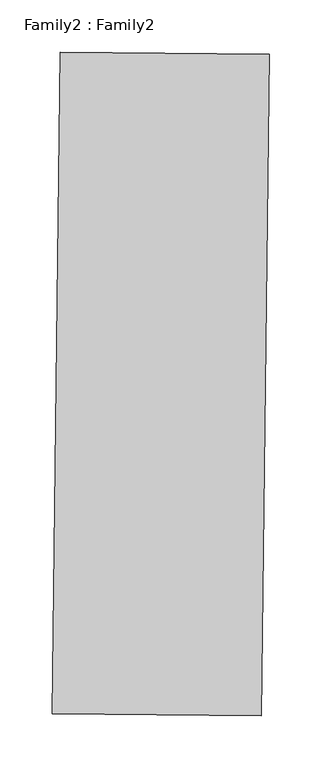
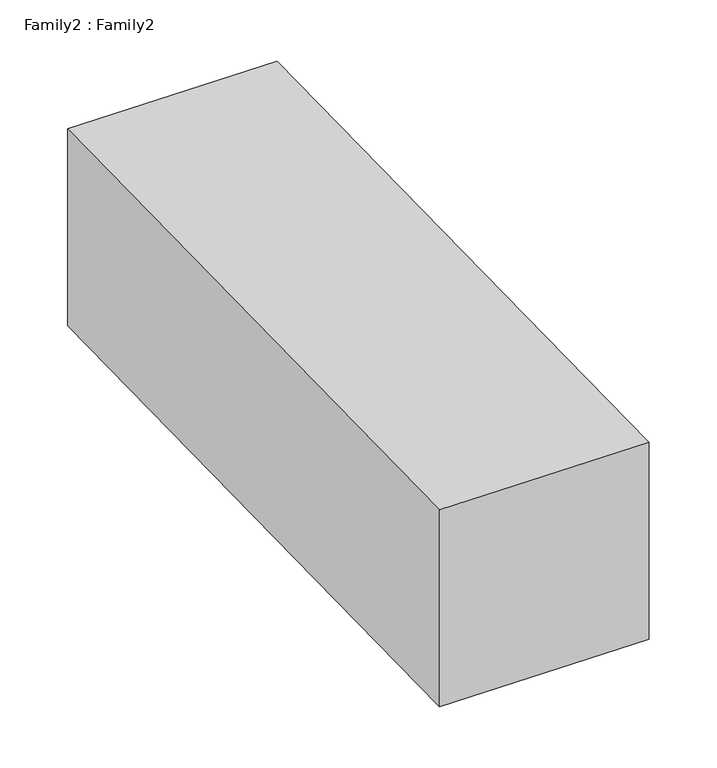
"""IFC4 building model written with IfcOpenShell, lengths in millimetres: proxy geometry, Family2 : Family2."""

import ifcopenshell
import ifcopenshell.guid

model = None  # the IFC model being written
_history = None  # IfcOwnerHistory: only IFC2X3 demands one
_inside = {}  # id of a spatial element -> (the spatial element, [elements in it])
_under = {}  # id of a project, library or spatial element -> (it, [spatial elements below it])
_declared = {}  # id of a project -> (the project, [libraries it declares])
_typed = {}  # id of a type object -> (the type object, [elements of that type])
_made_of = {}  # id of a material, layer set ... -> (it, [elements and type objects made of it])


def new_model(schema):
    """Start an empty IFC model of exactly this schema.

    Asked for "IFC4X3", IfcOpenShell would pick the latest addendum, in which some entities
    have other attributes; the version numbers below select the first issue.
    IFC2X3 requires an IfcOwnerHistory on every rooted entity: one is made here for all.
    """
    global model, _history
    if schema == "IFC4X3":
        model = ifcopenshell.file(schema_version=(4, 3, 0, 0))
    else:
        model = ifcopenshell.file(schema=schema)
    _inside.clear()
    _under.clear()
    _declared.clear()
    _typed.clear()
    _made_of.clear()
    _history = None
    if model.schema == "IFC2X3":
        org = make("IfcOrganization", Name="unknown")
        user = make(
            "IfcPersonAndOrganization",
            ThePerson=make("IfcPerson", FamilyName="unknown"),
            TheOrganization=org,
        )
        app = make(
            "IfcApplication",
            ApplicationDeveloper=org,
            Version="unknown",
            ApplicationFullName="unknown",
            ApplicationIdentifier="unknown",
        )
        _history = make(
            "IfcOwnerHistory",
            OwningUser=user,
            OwningApplication=app,
            ChangeAction="ADDED",
            CreationDate=0,
        )
    return model


def make(cls, **values):
    """One entity of the class cls with the attributes given. An attribute that is None is left unset."""
    return model.create_entity(
        cls, **{name: value for name, value in values.items() if value is not None}
    )


def rooted(cls, **values):
    """An entity with a GlobalId (a new one), such as an element, a storey or a relation."""
    return make(cls, GlobalId=ifcopenshell.guid.new(), OwnerHistory=_history, **values)


def si_unit(unit_type, name, prefix=None):
    """IfcSIUnit, for example si_unit("LENGTHUNIT", "METRE", prefix="MILLI")."""
    return make("IfcSIUnit", UnitType=unit_type, Prefix=prefix, Name=name)


def assignment(units):
    """IfcUnitAssignment: the units of a project."""
    return None if units is None else make("IfcUnitAssignment", Units=units)


def point(xyz):
    """IfcCartesianPoint."""
    return None if xyz is None else make("IfcCartesianPoint", Coordinates=xyz)


def direction(xyz):
    """IfcDirection."""
    return None if xyz is None else make("IfcDirection", DirectionRatios=xyz)


def frame(location, z_axis=None, x_axis=None):
    """IfcAxis2Placement3D, a coordinate frame: its origin and axes. An axis left out is left unset."""
    return make(
        "IfcAxis2Placement3D",
        Location=point(location),
        Axis=direction(z_axis),
        RefDirection=direction(x_axis),
    )


def origin():
    """The frame at (0, 0, 0) with its axes left unset."""
    return frame((0.0, 0.0, 0.0))


def place(relative_to, where):
    """IfcLocalPlacement: puts the frame where relative to a parent placement (None: the world)."""
    return make(
        "IfcLocalPlacement", PlacementRelTo=relative_to, RelativePlacement=where
    )


def context(
    kind, dimensions, precision=None, world=None, true_north=None, identifier=None
):
    """IfcGeometricRepresentationContext, for example the 3D "Model" context."""
    return make(
        "IfcGeometricRepresentationContext",
        ContextIdentifier=identifier,
        ContextType=kind,
        CoordinateSpaceDimension=dimensions,
        Precision=precision,
        WorldCoordinateSystem=world,
        TrueNorth=true_north,
    )


def project(units=None, contexts=None):
    """IfcProject with its units and contexts."""
    return rooted(
        "IfcProject",
        Name="project",
        RepresentationContexts=contexts,
        UnitsInContext=assignment(units),
    )


def spatial(cls, under=None, at=None, **own):
    """A site, building, storey or space (cls), placed at a placement, below another one or the project."""
    s = rooted(cls, ObjectPlacement=at, **own)
    if under is not None:
        _under.setdefault(under.id(), (under, []))[1].append(s)
    return s


def faces_of(points, faces, orient=None, outer=None):
    """IfcFace entities. A face is a list of loops; a loop is a list of indices into points, from 0.

    orient and outer hold one flag for each loop. By default every Orientation is true, the
    first loop of a face is its IfcFaceOuterBound and the others are IfcFaceBound.
    """
    made = []
    for i, loops in enumerate(faces):
        bounds = []
        for j, loop in enumerate(loops):
            is_outer = j == 0 if outer is None else outer[i][j]
            bounds.append(
                make(
                    "IfcFaceOuterBound" if is_outer else "IfcFaceBound",
                    Bound=make("IfcPolyLoop", Polygon=[points[k] for k in loop]),
                    Orientation=True if orient is None else orient[i][j],
                )
            )
        made.append(make("IfcFace", Bounds=bounds))
    return made


def faceted_brep(points, faces, orient=None, outer=None, voids=None):
    """IfcFacetedBrep: a solid bounded by flat faces; with voids (closed shells), ...WithVoids."""
    shared = [point(p) for p in points]
    hull = make("IfcClosedShell", CfsFaces=faces_of(shared, faces, orient, outer))
    if voids is None:
        return make("IfcFacetedBrep", Outer=hull)
    return make(
        "IfcFacetedBrepWithVoids",
        Outer=hull,
        Voids=[
            make(cls, CfsFaces=faces_of(shared, fs, o, b)) for cls, fs, o, b in voids
        ],
    )


def shape(context_of_items, identifier, shape_type, items):
    """IfcShapeRepresentation: the items that make up one representation, for example the "Body"."""
    return make(
        "IfcShapeRepresentation",
        ContextOfItems=context_of_items,
        RepresentationIdentifier=identifier,
        RepresentationType=shape_type,
        Items=items,
    )


def source(mapping_origin, context_of_items, identifier, shape_type, items):
    """IfcRepresentationMap: a shape defined once, which mapped items show again and again."""
    return make(
        "IfcRepresentationMap",
        MappingOrigin=mapping_origin,
        MappedRepresentation=shape(context_of_items, identifier, shape_type, items),
    )


def transform(
    local_origin,
    x_axis=None,
    y_axis=None,
    z_axis=None,
    scale=None,
    scale2=None,
    scale3=None,
    uniform=True,
):
    """IfcCartesianTransformationOperator3D, or its non-uniform kind. x_axis, y_axis, z_axis: its Axis1, 2, 3."""
    if uniform:
        return make(
            "IfcCartesianTransformationOperator3D",
            Axis1=direction(x_axis),
            Axis2=direction(y_axis),
            LocalOrigin=point(local_origin),
            Scale=scale,
            Axis3=direction(z_axis),
        )
    return make(
        "IfcCartesianTransformationOperator3DnonUniform",
        Axis1=direction(x_axis),
        Axis2=direction(y_axis),
        LocalOrigin=point(local_origin),
        Scale=scale,
        Axis3=direction(z_axis),
        Scale2=scale2,
        Scale3=scale3,
    )


def mapped(mapping_source, mapping_target):
    """IfcMappedItem: shows the shape of a source again, moved by a transform."""
    return make(
        "IfcMappedItem", MappingSource=mapping_source, MappingTarget=mapping_target
    )


def made_of(thing, what):
    """Note that an element or type object is made of a material, layer set ...; save() writes the relation."""
    if what is not None:
        _made_of.setdefault(what.id(), (what, []))[1].append(thing)
    return thing


def element(
    cls,
    number,
    at=None,
    inside=None,
    cuts=None,
    type_object=None,
    material=None,
    context=None,
    identifier="Body",
    shape_type=None,
    held_by="IfcProductDefinitionShape",
    body=None,
    shapes=None,
    **own,
):
    """One element of the class cls, such as IfcWall. Its Tag is "e" and its number.

    at: its placement. inside: the storey or other place that contains it. cuts: it is an
    opening in that element (IfcRelVoidsElement). A single representation is given by context,
    identifier, shape_type and body (its items); several are given by shapes. held_by: the class
    of the entity that holds the representations. save() writes the other relations.
    """
    e = rooted(cls, Tag="e%d" % number, ObjectPlacement=at, **own)
    if body is not None:
        shapes = [shape(context, identifier, shape_type, body)]
    if shapes is not None:
        e.Representation = make(held_by, Representations=shapes)
    if inside is not None:
        _inside.setdefault(inside.id(), (inside, []))[1].append(e)
    if cuts is not None:
        rooted(
            "IfcRelVoidsElement", RelatingBuildingElement=cuts, RelatedOpeningElement=e
        )
    if type_object is not None:
        _typed.setdefault(type_object.id(), (type_object, []))[1].append(e)
    return made_of(e, material)


def aggregate(whole, parts):
    """IfcRelAggregates: a whole, such as a stair, and the parts it consists of."""
    return rooted("IfcRelAggregates", RelatingObject=whole, RelatedObjects=parts)


def save(model, path):
    """Write the relations noted so far, then the file.

    IfcRelAggregates (storeys below a building ...), IfcRelContainedInSpatialStructure (elements
    in a storey), IfcRelDefinesByType, IfcRelAssociatesMaterial and IfcRelDeclares: one each for
    every whole, place, type object, material and project.
    """
    for whole, parts in _under.values():
        aggregate(whole, parts)
    for where, things in _inside.values():
        rooted(
            "IfcRelContainedInSpatialStructure",
            RelatedElements=things,
            RelatingStructure=where,
        )
    for kind, things in _typed.values():
        rooted("IfcRelDefinesByType", RelatedObjects=things, RelatingType=kind)
    for what, things in _made_of.values():
        rooted("IfcRelAssociatesMaterial", RelatedObjects=things, RelatingMaterial=what)
    for by, libraries in _declared.values():
        rooted("IfcRelDeclares", RelatingContext=by, RelatedDefinitions=libraries)
    model.write(path)


def family2_family2_042d18f2(model_context):
    return source(origin(), model_context, "Body", "Brep", [
        faceted_brep([(-3947.2035772, -6389.957857, 1.0945136), (-3947.2035772, -6389.957857, 201.0945136), (-3939.6392173, -5757.6422656, 202.060409), (-3939.6392173, -5757.6422656, 2.060409), (-3747.2123872, -6391.8350697, 201.0945136), (-3739.6480273, -5759.5194783, 202.060409), (-3747.2123872, -6391.8350697, 1.0945136), (-3739.6480273, -5759.5194783, 2.060409)], [[[0, 1, 2, 3]], [[1, 4, 5, 2]], [[4, 6, 7, 5]], [[6, 0, 3, 7]], [[3, 2, 5, 7]], [[0, 6, 4, 1]]]),
    ])


if __name__ == "__main__":
    model = new_model("IFC4")
    model_context = context("Model", 3, world=origin())
    ifc_project = project(units=[si_unit("LENGTHUNIT", "METRE", prefix="MILLI")], contexts=[model_context])
    site = spatial("IfcSite", under=ifc_project)
    building = spatial("IfcBuilding", under=site)
    placement = place(None, origin())
    family2_family2_shape = family2_family2_042d18f2(model_context)
    element("IfcBuildingElementProxy", 1, Name="Family2 : Family2", ObjectType="Family2 : Family2", at=placement, inside=building, context=model_context, shape_type="MappedRepresentation", body=[
        mapped(family2_family2_shape, transform((0.0, 0.0, 0.0), x_axis=(1.0, 0.0, 0.0), y_axis=(0.0, 1.0, 0.0), z_axis=(0.0, 0.0, 1.0))),
    ])
    save(model, "model.ifc")

# Revit data of these elements
# Type "Family2 : Family2"
#   Default Elevation = 0
